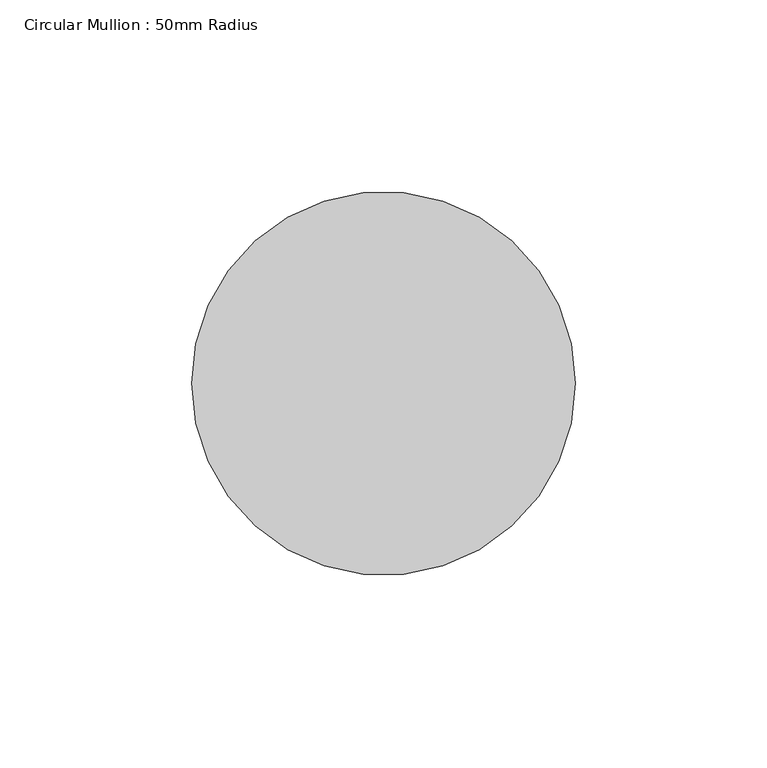
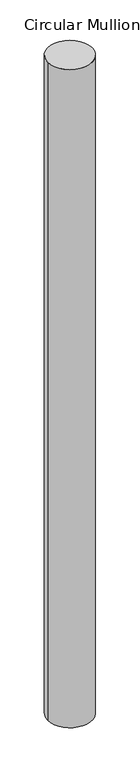
"""IFC4 building model written with IfcOpenShell, lengths in millimetres: member geometry, Circular Mullion : 50mm Radius."""

from ifc_helpers import new_model, si_unit, point, frame, origin, origin_2d, place, context, project, spatial, circle_curve, trimmed, segment, composite_curve, outline, extrude, source, transform, mapped, element, save


def circular_mullion_50mm_radius_b4bceef2(model_context):
    return source(origin(), model_context, "Body", "SweptSolid", [
        extrude(outline(composite_curve([segment(trimmed(circle_curve(origin_2d(), 50.0), [point((50.0, 0.0))], [point((-50.0, 0.0))], False, "CARTESIAN"), True, "CONTINUOUS"), segment(trimmed(circle_curve(origin_2d(), 50.0), [point((-50.0, 0.0))], [point((50.0, 0.0))], False, "CARTESIAN"), True, "CONTINUOUS")], self_intersect=False)), frame((0.0, 0.0, -1567.4592662), z_axis=(0.0, 0.0, 1.0), x_axis=(1.0, 0.0, 0.0)), (0.0, 0.0, 1.0), 1567.4592662),
    ])


if __name__ == "__main__":
    model = new_model("IFC4")
    model_context = context("Model", 3, world=origin())
    ifc_project = project(units=[si_unit("LENGTHUNIT", "METRE", prefix="MILLI")], contexts=[model_context])
    site = spatial("IfcSite", under=ifc_project)
    building = spatial("IfcBuilding", under=site)
    placement = place(None, origin())
    circular_mullion_50mm_radius_shape = circular_mullion_50mm_radius_b4bceef2(model_context)
    element("IfcMember", 1, ObjectType="Circular Mullion : 50mm Radius", at=placement, inside=building, context=model_context, shape_type="MappedRepresentation", body=[
        mapped(circular_mullion_50mm_radius_shape, transform((0.0, 0.0, 0.0), x_axis=(1.0, 0.0, 0.0), y_axis=(0.0, 1.0, 0.0), z_axis=(0.0, 0.0, 1.0))),
    ])
    save(model, "model.ifc")

# Revit data of these elements
# Type "Circular Mullion : 50mm Radius"
#   built-in parameter 1007350 = 0.164042 (stored number, unit not read)
# Element 1 (IfcMember, "Circular Mullion : 50mm Radius")
#   Materials on its faces: "Aluminium"
# Materials
#   "Aluminium": class "Metal", colour RGB 247 247 247, transparency 0, Description = "Aluminium 6061", Cost = 0
